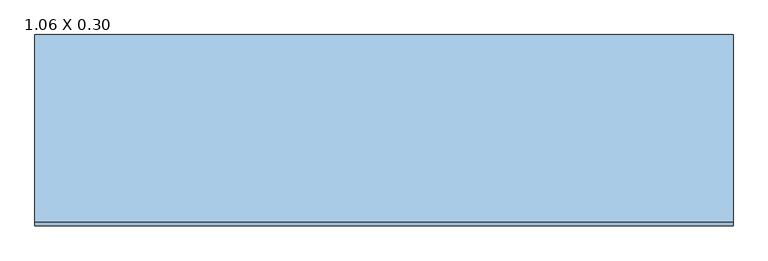
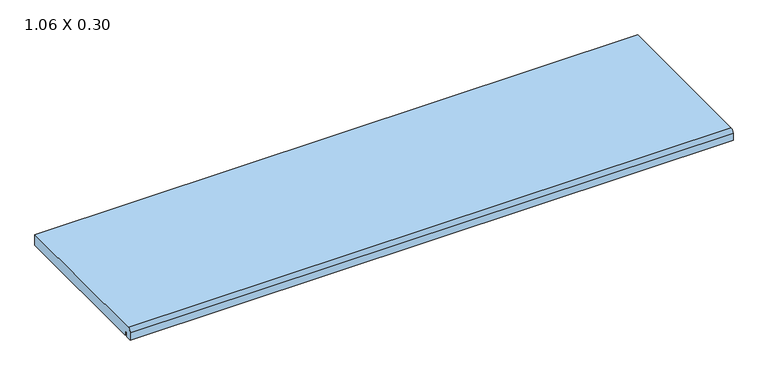
"""IFC4 building model written with IfcOpenShell, lengths in millimetres: window geometry, .CC_ND 300_PEDRA_PEITORIL RETO : 1.06 X 0.30."""

from ifc_helpers import new_model, si_unit, point, frame, frame_2d, origin, place, context, project, spatial, polyline, circle_curve, trimmed, segment, composite_curve, outline, extrude, source, transform, mapped, element, save


def window_1_06_x_0_30_38706416(model_context):
    return source(origin(), model_context, "Body", "SweptSolid", [
        extrude(outline(composite_curve([segment(polyline([(-132.5083081, 1480.0), (-132.5083081, 1488.1993124), (-137.2619526, 1488.1993124), (-137.2619526, 1480.0), (-148.0, 1480.0), (-148.0, 1493.3808343)]), True, "CONTINUOUS"), segment(trimmed(circle_curve(frame_2d((-141.3808343, 1493.3808343)), 6.6191657), [point((-148.0, 1493.3808343))], [point((-141.3808343, 1500.0))], False, "CARTESIAN"), True, "CONTINUOUS"), segment(polyline([(-141.3808343, 1500.0), (142.7, 1500.0), (142.7, 1480.0), (-132.5083081, 1480.0)]), True, "CONTINUOUS")], self_intersect=False)), frame((-530.0, 0.0, 0.0), z_axis=(1.0, 0.0, 0.0), x_axis=(0.0, 1.0, 0.0)), (0.0, 0.0, 1.0), 1060.0),
    ])


if __name__ == "__main__":
    model = new_model("IFC4")
    model_context = context("Model", 3, world=origin())
    ifc_project = project(units=[si_unit("LENGTHUNIT", "METRE", prefix="MILLI")], contexts=[model_context])
    site = spatial("IfcSite", under=ifc_project)
    building = spatial("IfcBuilding", under=site)
    placement = place(None, origin())
    window_1_06_x_0_30_shape = window_1_06_x_0_30_38706416(model_context)
    element("IfcWindow", 1, ObjectType=".CC_ND 300_PEDRA_PEITORIL RETO : 1.06 X 0.30", at=placement, inside=building, context=model_context, shape_type="MappedRepresentation", body=[
        mapped(window_1_06_x_0_30_shape, transform((0.0, 0.0, 0.0), x_axis=(1.0, 0.0, 0.0), y_axis=(0.0, 1.0, 0.0), z_axis=(0.0, 0.0, 1.0))),
    ])
    save(model, "model.ifc")

# Revit data of these elements
# Type ".CC_ND 300_PEDRA_PEITORIL RETO : 1.06 X 0.30"
#   Type Mark = "68"
#   Largura da pedra [instance default] = 0.26 m
#   Extensão interior peitoril [instance default] = 0.03 m
#   Extensão exterior peitoril [instance default] = 0.03 m
#   Espessura = 0.02 m
#   Comprimento = 1.06 m
#   Altura-padrão do peitoril = 1.48 m
#   Peitoril = .GRANITO_BRANCO_ITAUNAS
#   Rough Width = 0
#   Rough Height = 0
#   Height = 0
#   Wall Closure = (empty or 0)
#   Width = 0
# Element 1 (IfcWindow, ".CC_ND 300_PEDRA_PEITORIL RETO : 1.06 X 0.30")
#   Largura da pedra = 0.2907 m
#   Extensão interior peitoril = 0.0247 m
#   Materials on its faces: ".GRANITO_BRANCO_ITAUNAS"
# Materials
#   ".GRANITO_BRANCO_ITAUNAS": class ".CC_PEDRA REVEST.", colour RGB 202 195 174, transparency 0, Description = "Revestimento em granito", Cost = 0
